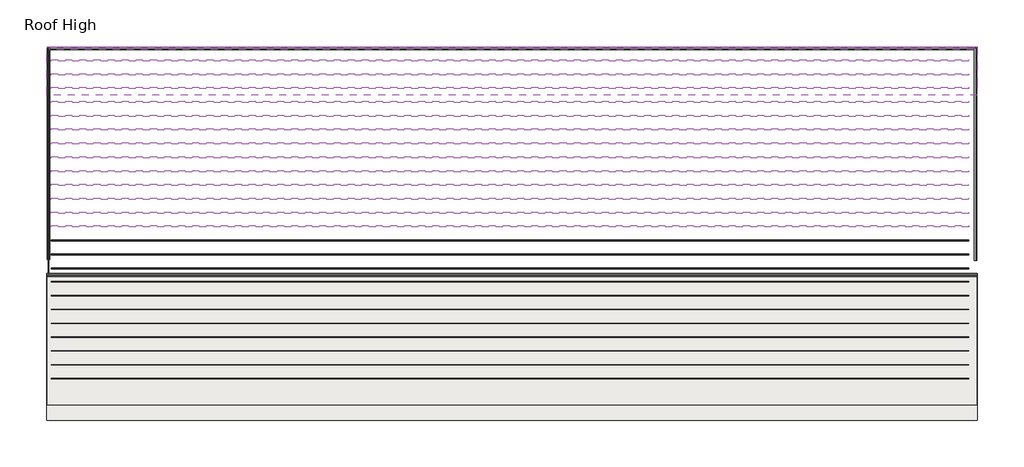
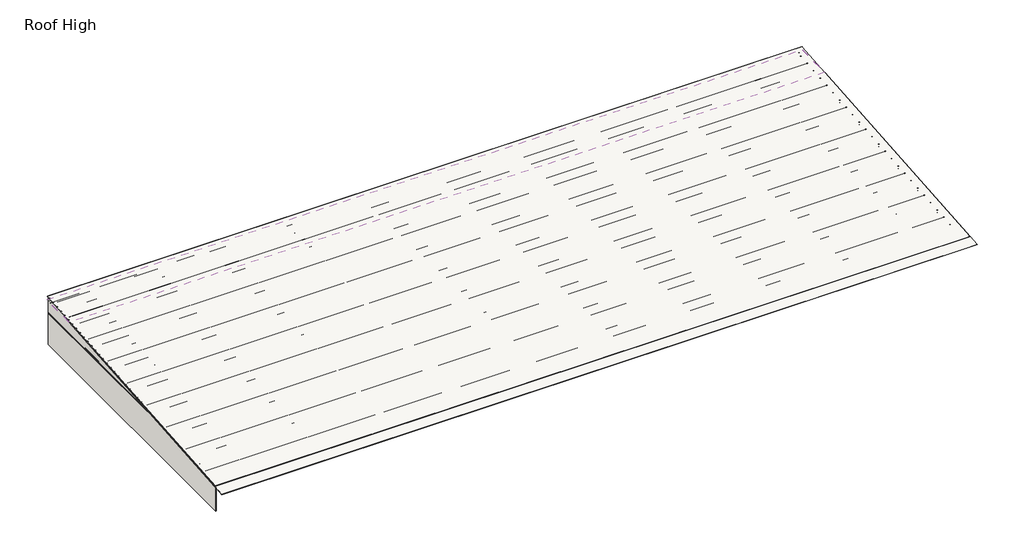
# One storey: 28 beams, 4 roofs, 1 proxy, 1 wall.
"""IFC4 building model written with IfcOpenShell, lengths in millimetres."""

import ifcopenshell
import ifcopenshell.guid

model = None  # the IFC model being written
_history = None  # IfcOwnerHistory: only IFC2X3 demands one
_inside = {}  # id of a spatial element -> (the spatial element, [elements in it])
_under = {}  # id of a project, library or spatial element -> (it, [spatial elements below it])
_declared = {}  # id of a project -> (the project, [libraries it declares])
_typed = {}  # id of a type object -> (the type object, [elements of that type])
_made_of = {}  # id of a material, layer set ... -> (it, [elements and type objects made of it])


def new_model(schema):
    """Start an empty IFC model of exactly this schema.

    Asked for "IFC4X3", IfcOpenShell would pick the latest addendum, in which some entities
    have other attributes; the version numbers below select the first issue.
    IFC2X3 requires an IfcOwnerHistory on every rooted entity: one is made here for all.
    """
    global model, _history
    if schema == "IFC4X3":
        model = ifcopenshell.file(schema_version=(4, 3, 0, 0))
    else:
        model = ifcopenshell.file(schema=schema)
    _inside.clear()
    _under.clear()
    _declared.clear()
    _typed.clear()
    _made_of.clear()
    _history = None
    if model.schema == "IFC2X3":
        org = make("IfcOrganization", Name="unknown")
        user = make(
            "IfcPersonAndOrganization",
            ThePerson=make("IfcPerson", FamilyName="unknown"),
            TheOrganization=org,
        )
        app = make(
            "IfcApplication",
            ApplicationDeveloper=org,
            Version="unknown",
            ApplicationFullName="unknown",
            ApplicationIdentifier="unknown",
        )
        _history = make(
            "IfcOwnerHistory",
            OwningUser=user,
            OwningApplication=app,
            ChangeAction="ADDED",
            CreationDate=0,
        )
    return model


def make(cls, **values):
    """One entity of the class cls with the attributes given. An attribute that is None is left unset."""
    return model.create_entity(
        cls, **{name: value for name, value in values.items() if value is not None}
    )


def rooted(cls, **values):
    """An entity with a GlobalId (a new one), such as an element, a storey or a relation."""
    return make(cls, GlobalId=ifcopenshell.guid.new(), OwnerHistory=_history, **values)


def si_unit(unit_type, name, prefix=None):
    """IfcSIUnit, for example si_unit("LENGTHUNIT", "METRE", prefix="MILLI")."""
    return make("IfcSIUnit", UnitType=unit_type, Prefix=prefix, Name=name)


def assignment(units):
    """IfcUnitAssignment: the units of a project."""
    return None if units is None else make("IfcUnitAssignment", Units=units)


def point(xyz):
    """IfcCartesianPoint."""
    return None if xyz is None else make("IfcCartesianPoint", Coordinates=xyz)


def direction(xyz):
    """IfcDirection."""
    return None if xyz is None else make("IfcDirection", DirectionRatios=xyz)


def frame(location, z_axis=None, x_axis=None):
    """IfcAxis2Placement3D, a coordinate frame: its origin and axes. An axis left out is left unset."""
    return make(
        "IfcAxis2Placement3D",
        Location=point(location),
        Axis=direction(z_axis),
        RefDirection=direction(x_axis),
    )


def frame_2d(location, x_axis=None):
    """IfcAxis2Placement2D, a coordinate frame in the plane: its origin and x axis."""
    return make(
        "IfcAxis2Placement2D", Location=point(location), RefDirection=direction(x_axis)
    )


def origin():
    """The frame at (0, 0, 0) with its axes left unset."""
    return frame((0.0, 0.0, 0.0))


def place(relative_to, where):
    """IfcLocalPlacement: puts the frame where relative to a parent placement (None: the world)."""
    return make(
        "IfcLocalPlacement", PlacementRelTo=relative_to, RelativePlacement=where
    )


def context(
    kind, dimensions, precision=None, world=None, true_north=None, identifier=None
):
    """IfcGeometricRepresentationContext, for example the 3D "Model" context."""
    return make(
        "IfcGeometricRepresentationContext",
        ContextIdentifier=identifier,
        ContextType=kind,
        CoordinateSpaceDimension=dimensions,
        Precision=precision,
        WorldCoordinateSystem=world,
        TrueNorth=true_north,
    )


def project(units=None, contexts=None):
    """IfcProject with its units and contexts."""
    return rooted(
        "IfcProject",
        Name="project",
        RepresentationContexts=contexts,
        UnitsInContext=assignment(units),
    )


def spatial(cls, under=None, at=None, **own):
    """A site, building, storey or space (cls), placed at a placement, below another one or the project."""
    s = rooted(cls, ObjectPlacement=at, **own)
    if under is not None:
        _under.setdefault(under.id(), (under, []))[1].append(s)
    return s


def polyline(points):
    """IfcPolyline through the points."""
    return make("IfcPolyline", Points=[point(p) for p in points])


def circle_curve(where, radius):
    """IfcCircle in the frame where."""
    return make("IfcCircle", Position=where, Radius=radius)


def trimmed(basis, trim1, trim2, sense, master):
    """IfcTrimmedCurve: the piece of a basis curve between two trims."""
    return make(
        "IfcTrimmedCurve",
        BasisCurve=basis,
        Trim1=trim1,
        Trim2=trim2,
        SenseAgreement=sense,
        MasterRepresentation=master,
    )


def segment(curve, same_sense, transition):
    """IfcCompositeCurveSegment."""
    return make(
        "IfcCompositeCurveSegment",
        Transition=transition,
        SameSense=same_sense,
        ParentCurve=curve,
    )


def composite_curve(segments, self_intersect=None):
    """IfcCompositeCurve: segments joined end to end."""
    return make("IfcCompositeCurve", Segments=segments, SelfIntersect=self_intersect)


def outline(outer, holes=None, kind="AREA"):
    """IfcArbitraryClosedProfileDef: a profile drawn as a closed curve; with holes, ...WithVoids."""
    if holes is None:
        return make("IfcArbitraryClosedProfileDef", ProfileType=kind, OuterCurve=outer)
    return make(
        "IfcArbitraryProfileDefWithVoids",
        ProfileType=kind,
        OuterCurve=outer,
        InnerCurves=holes,
    )


def extrude(swept, where, along, depth):
    """IfcExtrudedAreaSolid: the profile swept, set in the frame where, extruded along a direction by depth."""
    return make(
        "IfcExtrudedAreaSolid",
        SweptArea=swept,
        Position=where,
        ExtrudedDirection=direction(along),
        Depth=depth,
    )


def faces_of(points, faces, orient=None, outer=None):
    """IfcFace entities. A face is a list of loops; a loop is a list of indices into points, from 0.

    orient and outer hold one flag for each loop. By default every Orientation is true, the
    first loop of a face is its IfcFaceOuterBound and the others are IfcFaceBound.
    """
    made = []
    for i, loops in enumerate(faces):
        bounds = []
        for j, loop in enumerate(loops):
            is_outer = j == 0 if outer is None else outer[i][j]
            bounds.append(
                make(
                    "IfcFaceOuterBound" if is_outer else "IfcFaceBound",
                    Bound=make("IfcPolyLoop", Polygon=[points[k] for k in loop]),
                    Orientation=True if orient is None else orient[i][j],
                )
            )
        made.append(make("IfcFace", Bounds=bounds))
    return made


def faceted_brep(points, faces, orient=None, outer=None, voids=None):
    """IfcFacetedBrep: a solid bounded by flat faces; with voids (closed shells), ...WithVoids."""
    shared = [point(p) for p in points]
    hull = make("IfcClosedShell", CfsFaces=faces_of(shared, faces, orient, outer))
    if voids is None:
        return make("IfcFacetedBrep", Outer=hull)
    return make(
        "IfcFacetedBrepWithVoids",
        Outer=hull,
        Voids=[
            make(cls, CfsFaces=faces_of(shared, fs, o, b)) for cls, fs, o, b in voids
        ],
    )


def shape(context_of_items, identifier, shape_type, items):
    """IfcShapeRepresentation: the items that make up one representation, for example the "Body"."""
    return make(
        "IfcShapeRepresentation",
        ContextOfItems=context_of_items,
        RepresentationIdentifier=identifier,
        RepresentationType=shape_type,
        Items=items,
    )


def source(mapping_origin, context_of_items, identifier, shape_type, items):
    """IfcRepresentationMap: a shape defined once, which mapped items show again and again."""
    return make(
        "IfcRepresentationMap",
        MappingOrigin=mapping_origin,
        MappedRepresentation=shape(context_of_items, identifier, shape_type, items),
    )


def transform(
    local_origin,
    x_axis=None,
    y_axis=None,
    z_axis=None,
    scale=None,
    scale2=None,
    scale3=None,
    uniform=True,
):
    """IfcCartesianTransformationOperator3D, or its non-uniform kind. x_axis, y_axis, z_axis: its Axis1, 2, 3."""
    if uniform:
        return make(
            "IfcCartesianTransformationOperator3D",
            Axis1=direction(x_axis),
            Axis2=direction(y_axis),
            LocalOrigin=point(local_origin),
            Scale=scale,
            Axis3=direction(z_axis),
        )
    return make(
        "IfcCartesianTransformationOperator3DnonUniform",
        Axis1=direction(x_axis),
        Axis2=direction(y_axis),
        LocalOrigin=point(local_origin),
        Scale=scale,
        Axis3=direction(z_axis),
        Scale2=scale2,
        Scale3=scale3,
    )


def mapped(mapping_source, mapping_target):
    """IfcMappedItem: shows the shape of a source again, moved by a transform."""
    return make(
        "IfcMappedItem", MappingSource=mapping_source, MappingTarget=mapping_target
    )


def made_of(thing, what):
    """Note that an element or type object is made of a material, layer set ...; save() writes the relation."""
    if what is not None:
        _made_of.setdefault(what.id(), (what, []))[1].append(thing)
    return thing


def element(
    cls,
    number,
    at=None,
    inside=None,
    cuts=None,
    type_object=None,
    material=None,
    context=None,
    identifier="Body",
    shape_type=None,
    held_by="IfcProductDefinitionShape",
    body=None,
    shapes=None,
    **own,
):
    """One element of the class cls, such as IfcWall. Its Tag is "e" and its number.

    at: its placement. inside: the storey or other place that contains it. cuts: it is an
    opening in that element (IfcRelVoidsElement). A single representation is given by context,
    identifier, shape_type and body (its items); several are given by shapes. held_by: the class
    of the entity that holds the representations. save() writes the other relations.
    """
    e = rooted(cls, Tag="e%d" % number, ObjectPlacement=at, **own)
    if body is not None:
        shapes = [shape(context, identifier, shape_type, body)]
    if shapes is not None:
        e.Representation = make(held_by, Representations=shapes)
    if inside is not None:
        _inside.setdefault(inside.id(), (inside, []))[1].append(e)
    if cuts is not None:
        rooted(
            "IfcRelVoidsElement", RelatingBuildingElement=cuts, RelatedOpeningElement=e
        )
    if type_object is not None:
        _typed.setdefault(type_object.id(), (type_object, []))[1].append(e)
    return made_of(e, material)


def aggregate(whole, parts):
    """IfcRelAggregates: a whole, such as a stair, and the parts it consists of."""
    return rooted("IfcRelAggregates", RelatingObject=whole, RelatedObjects=parts)


def save(model, path):
    """Write the relations noted so far, then the file.

    IfcRelAggregates (storeys below a building ...), IfcRelContainedInSpatialStructure (elements
    in a storey), IfcRelDefinesByType, IfcRelAssociatesMaterial and IfcRelDeclares: one each for
    every whole, place, type object, material and project.
    """
    for whole, parts in _under.values():
        aggregate(whole, parts)
    for where, things in _inside.values():
        rooted(
            "IfcRelContainedInSpatialStructure",
            RelatedElements=things,
            RelatingStructure=where,
        )
    for kind, things in _typed.values():
        rooted("IfcRelDefinesByType", RelatedObjects=things, RelatingType=kind)
    for what, things in _made_of.values():
        rooted("IfcRelAssociatesMaterial", RelatedObjects=things, RelatingMaterial=what)
    for by, libraries in _declared.values():
        rooted("IfcRelDeclares", RelatingContext=by, RelatedDefinitions=libraries)
    model.write(path)


def beam_2a24e19f(model_context):
    return source(origin(), model_context, "Body", "SweptSolid", [
        extrude(outline(composite_curve([segment(polyline([(63.5, 127.0), (75.745104, 112.4068534), (73.6169367, 110.621109), (62.204539, 124.221875), (3.3005807, 124.221875)]), True, "CONTINUOUS"), segment(trimmed(circle_curve(frame_2d((3.3741066, 122.2381931)), 1.9850441), [point((3.3005807, 124.221875))], [point((1.3890625, 122.2381931))], True, "CARTESIAN"), True, "CONTINUOUS"), segment(polyline([(1.3890625, 122.2381931), (1.3890625, -122.2375)]), True, "CONTINUOUS"), segment(trimmed(circle_curve(frame_2d((-3.3734375, -122.2375)), 4.7625), [point((1.3890625, -122.2375))], [point((-3.3734375, -127.0))], False, "CARTESIAN"), True, "CONTINUOUS"), segment(polyline([(-3.3734375, -127.0), (-63.5, -127.0), (-75.745104, -112.4068534), (-73.6169367, -110.621109), (-62.204539, -124.221875), (-3.2694106, -124.221875)]), True, "CONTINUOUS"), segment(trimmed(circle_curve(frame_2d((-3.3748024, -122.2389339)), 1.9857399), [point((-3.2694106, -124.221875))], [point((-1.3890625, -122.2389339))], True, "CARTESIAN"), True, "CONTINUOUS"), segment(polyline([(-1.3890625, -122.2389339), (-1.3890625, 122.2375)]), True, "CONTINUOUS"), segment(trimmed(circle_curve(frame_2d((3.3734375, 122.2375)), 4.7625), [point((-1.3890625, 122.2375))], [point((3.3734375, 127.0))], False, "CARTESIAN"), True, "CONTINUOUS"), segment(polyline([(3.3734375, 127.0), (63.5, 127.0)]), True, "CONTINUOUS")], self_intersect=False)), frame((-40373.3, 0.0, 0.0), z_axis=(1.0, 0.0, 0.0), x_axis=(0.0, 1.0, 0.0)), (0.0, 0.0, 1.0), 80505.2999999),
    ])


def beam_abf8bc6d(model_context):
    return source(origin(), model_context, "Body", "SweptSolid", [
        extrude(outline(composite_curve([segment(polyline([(63.5, 127.0), (75.745104, 112.4068534), (73.6169367, 110.621109), (62.204539, 124.221875), (3.3005807, 124.221875)]), True, "CONTINUOUS"), segment(trimmed(circle_curve(frame_2d((3.3741066, 122.2381931)), 1.9850441), [point((3.3005807, 124.221875))], [point((1.3890625, 122.2381931))], True, "CARTESIAN"), True, "CONTINUOUS"), segment(polyline([(1.3890625, 122.2381931), (1.3890625, -122.2375)]), True, "CONTINUOUS"), segment(trimmed(circle_curve(frame_2d((-3.3734375, -122.2375)), 4.7625), [point((1.3890625, -122.2375))], [point((-3.3734375, -127.0))], False, "CARTESIAN"), True, "CONTINUOUS"), segment(polyline([(-3.3734375, -127.0), (-63.5, -127.0), (-75.745104, -112.4068534), (-73.6169367, -110.621109), (-62.204539, -124.221875), (-3.2694106, -124.221875)]), True, "CONTINUOUS"), segment(trimmed(circle_curve(frame_2d((-3.3748024, -122.2389339)), 1.9857399), [point((-3.2694106, -124.221875))], [point((-1.3890625, -122.2389339))], True, "CARTESIAN"), True, "CONTINUOUS"), segment(polyline([(-1.3890625, -122.2389339), (-1.3890625, 122.2375)]), True, "CONTINUOUS"), segment(trimmed(circle_curve(frame_2d((3.3734375, 122.2375)), 4.7625), [point((-1.3890625, 122.2375))], [point((3.3734375, 127.0))], False, "CARTESIAN"), True, "CONTINUOUS"), segment(polyline([(3.3734375, 127.0), (63.5, 127.0)]), True, "CONTINUOUS")], self_intersect=False)), frame((-40373.3, 0.0, 0.0), z_axis=(1.0, 0.0, 0.0), x_axis=(0.0, 1.0, 0.0)), (0.0, 0.0, 1.0), 80505.3),
    ])


def beam_1069c96b(model_context):
    return source(origin(), model_context, "Body", "SweptSolid", [
        extrude(outline(composite_curve([segment(polyline([(-63.5, 101.6), (-3.3734375, 101.6)]), True, "CONTINUOUS"), segment(trimmed(circle_curve(frame_2d((-3.3734375, 96.8375)), 4.7625), [point((-3.3734375, 101.6))], [point((1.3890625, 96.8375))], False, "CARTESIAN"), True, "CONTINUOUS"), segment(polyline([(1.3890625, 96.8375), (1.3890625, -96.8389339)]), True, "CONTINUOUS"), segment(trimmed(circle_curve(frame_2d((3.3748024, -96.8389339)), 1.9857399), [point((1.3890625, -96.8389339))], [point((3.2694106, -98.821875))], True, "CARTESIAN"), True, "CONTINUOUS"), segment(polyline([(3.2694106, -98.821875), (62.204539, -98.821875), (73.6169367, -85.221109), (75.745104, -87.0068534), (63.5, -101.6), (3.3734375, -101.6)]), True, "CONTINUOUS"), segment(trimmed(circle_curve(frame_2d((3.3734375, -96.8375)), 4.7625), [point((3.3734375, -101.6))], [point((-1.3890625, -96.8375))], False, "CARTESIAN"), True, "CONTINUOUS"), segment(polyline([(-1.3890625, -96.8375), (-1.3890625, 96.8381931)]), True, "CONTINUOUS"), segment(trimmed(circle_curve(frame_2d((-3.3741066, 96.8381931)), 1.9850441), [point((-1.3890625, 96.8381931))], [point((-3.3005807, 98.821875))], True, "CARTESIAN"), True, "CONTINUOUS"), segment(polyline([(-3.3005807, 98.821875), (-62.204539, 98.821875), (-73.6169367, 85.221109), (-75.745104, 87.0068534), (-63.5, 101.6)]), True, "CONTINUOUS")], self_intersect=False)), frame((-40602.569726, 0.0, 0.0), z_axis=(1.0, 0.0, 0.0), x_axis=(0.0, 1.0, 0.0)), (0.0, 0.0, 1.0), 81057.5019525),
    ])


def beam_935b8cdd(model_context):
    return source(origin(), model_context, "Body", "SweptSolid", [
        extrude(outline(composite_curve([segment(polyline([(63.5, 101.6), (75.745104, 87.0068534), (73.6169367, 85.221109), (62.204539, 98.821875), (3.3005807, 98.821875)]), True, "CONTINUOUS"), segment(trimmed(circle_curve(frame_2d((3.3741066, 96.8381931)), 1.9850441), [point((3.3005807, 98.821875))], [point((1.3890625, 96.8381931))], True, "CARTESIAN"), True, "CONTINUOUS"), segment(polyline([(1.3890625, 96.8381931), (1.3890625, -96.8375)]), True, "CONTINUOUS"), segment(trimmed(circle_curve(frame_2d((-3.3734375, -96.8375)), 4.7625), [point((1.3890625, -96.8375))], [point((-3.3734375, -101.6))], False, "CARTESIAN"), True, "CONTINUOUS"), segment(polyline([(-3.3734375, -101.6), (-63.5, -101.6), (-75.745104, -87.0068534), (-73.6169367, -85.221109), (-62.204539, -98.821875), (-3.2694106, -98.821875)]), True, "CONTINUOUS"), segment(trimmed(circle_curve(frame_2d((-3.3748024, -96.8389339)), 1.9857399), [point((-3.2694106, -98.821875))], [point((-1.3890625, -96.8389339))], True, "CARTESIAN"), True, "CONTINUOUS"), segment(polyline([(-1.3890625, -96.8389339), (-1.3890625, 96.8375)]), True, "CONTINUOUS"), segment(trimmed(circle_curve(frame_2d((3.3734375, 96.8375)), 4.7625), [point((-1.3890625, 96.8375))], [point((3.3734375, 101.6))], False, "CARTESIAN"), True, "CONTINUOUS"), segment(polyline([(3.3734375, 101.6), (63.5, 101.6)]), True, "CONTINUOUS")], self_intersect=False)), frame((-9323.6355469, 0.0, 0.0), z_axis=(1.0, 0.0, 0.0), x_axis=(0.0, 1.0, 0.0)), (0.0, 0.0, 1.0), 18647.2710937),
    ])


def beam_7c8f2e1c(model_context):
    return source(origin(), model_context, "Body", "SweptSolid", [
        extrude(outline(composite_curve([segment(polyline([(-63.5, 101.6), (-3.3734375, 101.6)]), True, "CONTINUOUS"), segment(trimmed(circle_curve(frame_2d((-3.3734375, 96.8375)), 4.7625), [point((-3.3734375, 101.6))], [point((1.3890625, 96.8375))], False, "CARTESIAN"), True, "CONTINUOUS"), segment(polyline([(1.3890625, 96.8375), (1.3890625, -96.8389339)]), True, "CONTINUOUS"), segment(trimmed(circle_curve(frame_2d((3.3748024, -96.8389339)), 1.9857399), [point((1.3890625, -96.8389339))], [point((3.2694106, -98.821875))], True, "CARTESIAN"), True, "CONTINUOUS"), segment(polyline([(3.2694106, -98.821875), (62.204539, -98.821875), (73.6169367, -85.221109), (75.745104, -87.0068534), (63.5, -101.6), (3.3734375, -101.6)]), True, "CONTINUOUS"), segment(trimmed(circle_curve(frame_2d((3.3734375, -96.8375)), 4.7625), [point((3.3734375, -101.6))], [point((-1.3890625, -96.8375))], False, "CARTESIAN"), True, "CONTINUOUS"), segment(polyline([(-1.3890625, -96.8375), (-1.3890625, 96.8381931)]), True, "CONTINUOUS"), segment(trimmed(circle_curve(frame_2d((-3.3741066, 96.8381931)), 1.9850441), [point((-1.3890625, 96.8381931))], [point((-3.3005807, 98.821875))], True, "CARTESIAN"), True, "CONTINUOUS"), segment(polyline([(-3.3005807, 98.821875), (-62.204539, 98.821875), (-73.6169367, 85.221109), (-75.745104, 87.0068534), (-63.5, 101.6)]), True, "CONTINUOUS")], self_intersect=False)), frame((-9209.8316406, 0.0, 0.0), z_axis=(1.0, 0.0, 0.0), x_axis=(0.0, 1.0, 0.0)), (0.0, 0.0, 1.0), 18529.7960937),
    ])


def beam_4e68f0c2(model_context):
    return source(origin(), model_context, "Body", "SweptSolid", [
        extrude(outline(composite_curve([segment(polyline([(-63.5, 101.6), (-3.3734375, 101.6)]), True, "CONTINUOUS"), segment(trimmed(circle_curve(frame_2d((-3.3734375, 96.8375)), 4.7625), [point((-3.3734375, 101.6))], [point((1.3890625, 96.8375))], False, "CARTESIAN"), True, "CONTINUOUS"), segment(polyline([(1.3890625, 96.8375), (1.3890625, -96.8389339)]), True, "CONTINUOUS"), segment(trimmed(circle_curve(frame_2d((3.3748024, -96.8389339)), 1.9857399), [point((1.3890625, -96.8389339))], [point((3.2694106, -98.821875))], True, "CARTESIAN"), True, "CONTINUOUS"), segment(polyline([(3.2694106, -98.821875), (62.204539, -98.821875), (73.6169367, -85.221109), (75.745104, -87.0068534), (63.5, -101.6), (3.3734375, -101.6)]), True, "CONTINUOUS"), segment(trimmed(circle_curve(frame_2d((3.3734375, -96.8375)), 4.7625), [point((3.3734375, -101.6))], [point((-1.3890625, -96.8375))], False, "CARTESIAN"), True, "CONTINUOUS"), segment(polyline([(-1.3890625, -96.8375), (-1.3890625, 96.8381931)]), True, "CONTINUOUS"), segment(trimmed(circle_curve(frame_2d((-3.3741066, 96.8381931)), 1.9850441), [point((-1.3890625, 96.8381931))], [point((-3.3005807, 98.821875))], True, "CARTESIAN"), True, "CONTINUOUS"), segment(polyline([(-3.3005807, 98.821875), (-62.204539, 98.821875), (-73.6169367, 85.221109), (-75.745104, 87.0068534), (-63.5, 101.6)]), True, "CONTINUOUS")], self_intersect=False)), frame((-40615.2697266, 0.0, 0.0), z_axis=(1.0, 0.0, 0.0), x_axis=(0.0, 1.0, 0.0)), (0.0, 0.0, 1.0), 81070.2019531),
    ])


model = new_model("IFC4")

# Units and contexts
model_context = context("Model", 3, world=origin())
ifc_project = project(units=[si_unit("LENGTHUNIT", "METRE", prefix="MILLI")], contexts=[model_context])

# Site, building, storey
site = spatial("IfcSite", under=ifc_project)
building = spatial("IfcBuilding", under=site)
storey = spatial("IfcBuildingStorey", under=building, Name="Roof High", Elevation=8737.6)

# Beams
placement = place(None, origin())
beam_shape = beam_2a24e19f(model_context)
element("IfcBeam", 1, ObjectType="Girt_Z : 10\"D", at=placement, inside=storey, context=model_context, shape_type="MappedRepresentation", body=[
    mapped(beam_shape, transform((619401.6117241, -537915.7766687, 11367.5039356), x_axis=(1.0, 0.0, 0.0), y_axis=(0.0, 0.996545758244879, 0.08304547985374816), z_axis=(0.0, -0.08304547985374816, 0.996545758244879))),
])
element("IfcBeam", 2, ObjectType="Girt_Z : 10\"D", at=placement, inside=storey, context=model_context, shape_type="MappedRepresentation", body=[
    mapped(beam_shape, transform((619401.6117241, -539130.7652571, 11266.2548865), x_axis=(1.0, 0.0, 0.0), y_axis=(0.0, 0.996545758244879, 0.08304547985374816), z_axis=(0.0, -0.08304547985374816, 0.996545758244879))),
])
element("IfcBeam", 3, ObjectType="Girt_Z : 10\"D", at=placement, inside=storey, context=model_context, shape_type="MappedRepresentation", body=[
    mapped(beam_shape, transform((619401.6117241, -540345.7538456, 11165.0058375), x_axis=(1.0, 0.0, 0.0), y_axis=(0.0, 0.996545758244879, 0.08304547985374816), z_axis=(0.0, -0.08304547985374816, 0.996545758244879))),
])
element("IfcBeam", 4, ObjectType="Girt_Z : 10\"D", at=placement, inside=storey, context=model_context, shape_type="MappedRepresentation", body=[
    mapped(beam_shape, transform((619401.6117241, -541560.742434, 11063.7567885), x_axis=(1.0, 0.0, 0.0), y_axis=(0.0, 0.996545758244879, 0.08304547985374816), z_axis=(0.0, -0.08304547985374816, 0.996545758244879))),
])
element("IfcBeam", 5, ObjectType="Girt_Z : 10\"D", at=placement, inside=storey, context=model_context, shape_type="MappedRepresentation", body=[
    mapped(beam_shape, transform((619401.6117241, -542775.7310225, 10962.5077394), x_axis=(1.0, 0.0, 0.0), y_axis=(0.0, 0.996545758244879, 0.08304547985374816), z_axis=(0.0, -0.08304547985374816, 0.996545758244879))),
])
element("IfcBeam", 6, ObjectType="Girt_Z : 10\"D", at=placement, inside=storey, context=model_context, shape_type="MappedRepresentation", body=[
    mapped(beam_shape, transform((619401.6117241, -543990.7196109, 10861.2586904), x_axis=(1.0, 0.0, 0.0), y_axis=(0.0, 0.996545758244879, 0.08304547985374816), z_axis=(0.0, -0.08304547985374816, 0.996545758244879))),
])
element("IfcBeam", 7, ObjectType="Girt_Z : 10\"D", at=placement, inside=storey, context=model_context, shape_type="MappedRepresentation", body=[
    mapped(beam_shape, transform((619401.6117241, -545205.7081994, 10760.0096414), x_axis=(1.0, 0.0, 0.0), y_axis=(0.0, 0.996545758244879, 0.08304547985374816), z_axis=(0.0, -0.08304547985374816, 0.996545758244879))),
])
element("IfcBeam", 8, ObjectType="Girt_Z : 10\"D", at=placement, inside=storey, context=model_context, shape_type="MappedRepresentation", body=[
    mapped(beam_shape, transform((619401.6117241, -546420.6967878, 10658.7605923), x_axis=(1.0, 0.0, 0.0), y_axis=(0.0, 0.996545758244879, 0.08304547985374816), z_axis=(0.0, -0.08304547985374816, 0.996545758244879))),
])
element("IfcBeam", 9, ObjectType="Girt_Z : 10\"D", at=placement, inside=storey, context=model_context, shape_type="MappedRepresentation", body=[
    mapped(beam_shape, transform((619401.6117241, -547635.6853763, 10557.5115433), x_axis=(1.0, 0.0, 0.0), y_axis=(0.0, 0.996545758244879, 0.08304547985374816), z_axis=(0.0, -0.08304547985374816, 0.996545758244879))),
])
element("IfcBeam", 10, ObjectType="Girt_Z : 10\"D", at=placement, inside=storey, context=model_context, shape_type="MappedRepresentation", body=[
    mapped(beam_shape, transform((619401.6117241, -548850.6739647, 10456.2624942), x_axis=(1.0, 0.0, 0.0), y_axis=(0.0, 0.996545758244879, 0.08304547985374816), z_axis=(0.0, -0.08304547985374816, 0.996545758244879))),
])
element("IfcBeam", 11, ObjectType="Girt_Z : 10\"D", at=placement, inside=storey, context=model_context, shape_type="MappedRepresentation", body=[
    mapped(beam_shape, transform((619401.6117241, -550065.6625532, 10355.0134452), x_axis=(1.0, 0.0, 0.0), y_axis=(0.0, 0.996545758244879, 0.08304547985374816), z_axis=(0.0, -0.08304547985374816, 0.996545758244879))),
])
element("IfcBeam", 12, ObjectType="Girt_Z : 10\"D", at=placement, inside=storey, context=model_context, shape_type="MappedRepresentation", body=[
    mapped(beam_shape, transform((619401.6117241, -551280.6511416, 10253.7643962), x_axis=(1.0, 0.0, 0.0), y_axis=(0.0, 0.996545758244879, 0.08304547985374816), z_axis=(0.0, -0.08304547985374816, 0.996545758244879))),
])
element("IfcBeam", 13, ObjectType="Girt_Z : 10\"D", at=placement, inside=storey, context=model_context, shape_type="MappedRepresentation", body=[
    mapped(beam_shape, transform((619401.6117241, -552495.6397301, 10152.5153471), x_axis=(1.0, 0.0, 0.0), y_axis=(0.0, 0.996545758244879, 0.08304547985374816), z_axis=(0.0, -0.08304547985374816, 0.996545758244879))),
])
element("IfcBeam", 14, ObjectType="Girt_Z : 10\"D", at=placement, inside=storey, context=model_context, shape_type="MappedRepresentation", body=[
    mapped(beam_shape, transform((619401.6117241, -553710.6283185, 10051.2662981), x_axis=(1.0, 0.0, 0.0), y_axis=(0.0, 0.996545758244879, 0.08304547985374816), z_axis=(0.0, -0.08304547985374816, 0.996545758244879))),
])
element("IfcBeam", 15, ObjectType="Girt_Z : 10\"D", at=placement, inside=storey, context=model_context, shape_type="MappedRepresentation", body=[
    mapped(beam_shape, transform((619401.6117241, -554925.616907, 9950.0172491), x_axis=(1.0, 0.0, 0.0), y_axis=(0.0, 0.996545758244879, 0.08304547985374816), z_axis=(0.0, -0.08304547985374816, 0.996545758244879))),
])
element("IfcBeam", 16, ObjectType="Girt_Z : 10\"D", at=placement, inside=storey, context=model_context, shape_type="MappedRepresentation", body=[
    mapped(beam_shape, transform((619401.6117241, -556140.6054954, 9848.7682), x_axis=(1.0, 0.0, 0.0), y_axis=(0.0, 0.996545758244879, 0.08304547985374816), z_axis=(0.0, -0.08304547985374816, 0.996545758244879))),
])
element("IfcBeam", 17, ObjectType="Girt_Z : 10\"D", at=placement, inside=storey, context=model_context, shape_type="MappedRepresentation", body=[
    mapped(beam_shape, transform((619401.6117241, -557355.5940839, 9747.519151), x_axis=(1.0, 0.0, 0.0), y_axis=(0.0, 0.996545758244879, 0.08304547985374816), z_axis=(0.0, -0.08304547985374816, 0.996545758244879))),
])
element("IfcBeam", 18, ObjectType="Girt_Z : 10\"D", at=placement, inside=storey, context=model_context, shape_type="MappedRepresentation", body=[
    mapped(beam_shape, transform((619401.6117241, -558570.5826724, 9646.2701019), x_axis=(1.0, 0.0, 0.0), y_axis=(0.0, 0.996545758244879, 0.08304547985374816), z_axis=(0.0, -0.08304547985374816, 0.996545758244879))),
])
element("IfcBeam", 19, ObjectType="Girt_Z : 10\"D", at=placement, inside=storey, context=model_context, shape_type="MappedRepresentation", body=[
    mapped(beam_shape, transform((619401.6117241, -559785.5712608, 9545.0210529), x_axis=(1.0, 0.0, 0.0), y_axis=(0.0, 0.996545758244879, 0.08304547985374816), z_axis=(0.0, -0.08304547985374816, 0.996545758244879))),
])
element("IfcBeam", 20, ObjectType="Girt_Z : 10\"D", at=placement, inside=storey, context=model_context, shape_type="MappedRepresentation", body=[
    mapped(beam_shape, transform((619401.6117241, -561000.5598493, 9443.7720039), x_axis=(1.0, 0.0, 0.0), y_axis=(0.0, 0.996545758244879, 0.08304547985374816), z_axis=(0.0, -0.08304547985374816, 0.996545758244879))),
])
beam_2_shape = beam_abf8bc6d(model_context)
element("IfcBeam", 21, ObjectType="Girt_Z : 10\"D", at=placement, inside=storey, context=model_context, shape_type="MappedRepresentation", body=[
    mapped(beam_2_shape, transform((619401.6117241, -562215.5484377, 9342.5229548), x_axis=(1.0, 0.0, 0.0), y_axis=(0.0, 0.996545758244879, 0.08304547985374816), z_axis=(0.0, -0.08304547985374816, 0.996545758244879))),
])
element("IfcBeam", 22, ObjectType="Girt_Z : 10\"D", at=placement, inside=storey, context=model_context, shape_type="MappedRepresentation", body=[
    mapped(beam_2_shape, transform((619401.6117241, -563430.5370262, 9241.2739058), x_axis=(1.0, 0.0, 0.0), y_axis=(0.0, 0.996545758244879, 0.08304547985374816), z_axis=(0.0, -0.08304547985374816, 0.996545758244879))),
])
element("IfcBeam", 23, ObjectType="Girt_Z : 10\"D", at=placement, inside=storey, context=model_context, shape_type="MappedRepresentation", body=[
    mapped(beam_2_shape, transform((619401.6117241, -564645.5256146, 9140.0248567), x_axis=(1.0, 0.0, 0.0), y_axis=(0.0, 0.996545758244879, 0.08304547985374816), z_axis=(0.0, -0.08304547985374816, 0.996545758244879))),
])
element("IfcBeam", 24, ObjectType="Girt_Z : 10\"D", at=placement, inside=storey, context=model_context, shape_type="MappedRepresentation", body=[
    mapped(beam_2_shape, transform((619401.6117241, -565860.5142031, 9038.7758077), x_axis=(1.0, 0.0, 0.0), y_axis=(0.0, 0.996545758244879, 0.08304547985374816), z_axis=(0.0, -0.08304547985374816, 0.996545758244879))),
])
beam_3_shape = beam_1069c96b(model_context)
element("IfcBeam", 25, ObjectType="Girt_Z : 8\"D", at=placement, inside=storey, context=model_context, shape_type="MappedRepresentation", body=[
    mapped(beam_3_shape, transform((619520.0044974, -536855.7413841, 9753.6), x_axis=(1.0000000000000002, 0.0, 0.0), y_axis=(0.0, 0.0, 1.0000000000000002), z_axis=(0.0, -1.0000000000000002, 0.0))),
])
beam_4_shape = beam_935b8cdd(model_context)
element("IfcBeam", 26, ObjectType="Girt_Z : 8\"D", at=placement, inside=storey, context=model_context, shape_type="MappedRepresentation", body=[
    mapped(beam_4_shape, transform((660105.1117239, -546179.376931, 9753.6), x_axis=(0.0, 1.0000000000000002, 0.0), y_axis=(0.0, 0.0, -1.0000000000000002), z_axis=(-1.0000000000000002, 0.0, 0.0))),
])
beam_5_shape = beam_7c8f2e1c(model_context)
element("IfcBeam", 27, ObjectType="Girt_Z : 8\"D", at=placement, inside=storey, context=model_context, shape_type="MappedRepresentation", body=[
    mapped(beam_5_shape, transform((578803.1347708, -546175.7058372, 9753.6), x_axis=(0.0, 1.0000000000000002, 0.0), y_axis=(0.0, 0.0, 1.0000000000000002), z_axis=(1.0000000000000002, 0.0, 0.0))),
])
beam_6_shape = beam_4e68f0c2(model_context)
element("IfcBeam", 28, ObjectType="Girt_Z : 8\"D", at=placement, inside=storey, context=model_context, shape_type="MappedRepresentation", body=[
    mapped(beam_6_shape, transform((619520.0044974, -536855.7413841, 10972.8), x_axis=(1.0000000000000002, 0.0, 0.0), y_axis=(0.0, 0.0, 1.0000000000000002), z_axis=(0.0, -1.0000000000000002, 0.0))),
])

# Proxy
element("IfcBuildingElementProxy", 29, Name="Wall Sweeps", at=placement, inside=storey, context=model_context, shape_type="SweptSolid", body=[
    extrude(outline(polyline([(-536747.7913841, 11605.3516632), (-536693.7909841, 11605.3516632), (-536693.7909841, 11533.3680632), (-536696.9659841, 11533.3680632), (-536696.9659841, 11534.9555632), (-536695.3784841, 11534.9555632), (-536695.3784841, 11603.7641632), (-536746.2038841, 11603.7641632), (-536746.2038841, 11514.9403632), (-536740.3872841, 11514.9403632), (-536740.3872841, 11519.7028632), (-536738.7997841, 11519.7028632), (-536738.7997841, 11513.3528632), (-536747.7913841, 11513.3528632), (-536747.7913841, 11605.3516632)])), frame((578766.7848054, 0.0, 0.0), z_axis=(1.0, 0.0, 0.0), x_axis=(0.0, 1.0, 0.0)), (0.0, 0.0, 1.0), 81475.5021585),
])

# Roofs
element("IfcRoof", 30, ObjectType="arcoPlus_6124_with_IR", at=placement, inside=storey, context=model_context, shape_type="SweptSolid", body=[
    extrude(outline(polyline([(-568168.5413949, 9002.8608333), (-536724.1414187, 11623.227498), (-536724.1414187, 11611.1804157), (-568168.5413949, 8990.813751), (-568168.5413949, 9002.8608333)])), frame((578668.83476, 0.0, 0.0), z_axis=(1.0, 0.0, 0.0), x_axis=(0.0, 1.0, 0.0)), (0.0, 0.0, 1.0), 81557.8769747),
])
element("IfcRoof", 31, ObjectType="arcoPlus_6124_with_IR", at=placement, inside=storey, context=model_context, shape_type="SweptSolid", body=[
    extrude(outline(polyline([(-568204.1165841, 8982.9629009), (-540960.9909841, 11253.2233675), (-540960.9909841, 11241.1762853), (-568204.1165841, 8970.9158186), (-568204.1165841, 8982.9629009)])), frame((578625.3347708, 0.0, 0.0), z_axis=(1.0, 0.0, 0.0), x_axis=(0.0, 1.0, 0.0)), (0.0, 0.0, 1.0), 81657.5769531),
])
element("IfcRoof", 32, ObjectType="Metal Roof - Structural Standing Seam", at=placement, inside=storey, context=model_context, shape_type="SweptSolid", body=[
    extrude(outline(polyline([(-540960.9909841, 11253.2233675), (-536693.7909841, 11608.8233675), (-536693.7909841, 11596.7762853), (-540960.9909841, 11241.1762853), (-540960.9909841, 11253.2233675)])), frame((578625.3347708, 0.0, 0.0), z_axis=(1.0, 0.0, 0.0), x_axis=(0.0, 1.0, 0.0)), (0.0, 0.0, 1.0), 81657.5769531),
])
element("IfcRoof", 33, ObjectType="Shading Material", at=placement, inside=storey, context=model_context, shape_type="SweptSolid", body=[
    extrude(outline(polyline([(-569520.1413841, 8873.2941675), (-568178.5413495, 8985.0941704), (-568178.5413495, 8973.0470881), (-569520.1413841, 8861.2470853), (-569520.1413841, 8873.2941675)])), frame((578625.3347708, 0.0, 0.0), z_axis=(1.0, 0.0, 0.0), x_axis=(0.0, 1.0, 0.0)), (0.0, 0.0, 1.0), 81657.5769531),
])

# Wall
element("IfcWall", 34, ObjectType="arcoPlus - 547", at=placement, inside=storey, context=model_context, shape_type="Brep", body=[
    faceted_brep([(578766.7848054, -536738.5661041, 6097.5875), (578766.7848054, -568164.1166641, 6097.5875), (578766.7848054, -568164.1166641, 8974.2491453), (578766.7848054, -536747.7913841, 11592.2762519), (578766.7848054, -536747.7913841, 11513.3528632), (578766.7848054, -536738.7997841, 11513.3528632), (578766.7848054, -536738.7997841, 11519.7028632), (578766.7848054, -536740.3872841, 11519.7028632), (578766.7848054, -536740.3872841, 11514.9403632), (578766.7848054, -536746.2038841, 11514.9403632), (578766.7848054, -536746.2038841, 11592.4085436), (578766.7848054, -536738.5661041, 11593.0450253), (578766.7848054, -536738.5661041, 11576.8528632), (578806.7847254, -568164.1166641, 6097.5875), (578806.7847254, -536738.5661041, 6097.5875), (578806.7847254, -536738.5661041, 11593.0450253), (578806.7847254, -536746.2038841, 11592.4085436), (578806.7847254, -536746.2038841, 11514.9403632), (578806.7847254, -536740.3872841, 11514.9403632), (578806.7847254, -536740.3872841, 11519.7028632), (578806.7847254, -536738.7997841, 11519.7028632), (578806.7847254, -536738.7997841, 11513.3528632), (578806.7847254, -536747.7913841, 11513.3528632), (578806.7847254, -536747.7913841, 11592.2762519), (578806.7847254, -568164.1166641, 8974.2491453)], [[[0, 1, 2, 3, 4, 5, 6, 7, 8, 9, 10, 11, 12]], [[13, 14, 15, 16, 17, 18, 19, 20, 21, 22, 23, 24]], [[2, 24, 23, 3]], [[15, 11, 10, 16]], [[1, 0, 14, 13]], [[24, 2, 1, 13]], [[11, 15, 14, 0, 12]], [[22, 4, 3, 23]], [[4, 22, 21, 5]], [[5, 21, 20, 6]], [[6, 20, 19, 7]], [[7, 19, 18, 8]], [[8, 18, 17, 9]], [[9, 17, 16, 10]]]),
])

save(model, "model.ifc")

# Revit data of these elements
# Project information
#   Project Issue Date = "Issue Date"
#   Project Status = "Project Status"
#   Client Name = "Xcel Fitness"
#   Project Address = "Enter address here"
#   Project Name = "Xcel Sports Complex"
#   Project Number = "Project Number"
# Grids (mm)
#   "1": line (579028.312, -472874.843) -> (579028.312, -580344.522)
#   "2": line (586368.912, -472874.843) -> (586368.912, -580344.522)
#   "3": line (593709.512, -472874.843) -> (593709.512, -580344.522)
#   "4": line (601050.112, -472874.843) -> (601050.112, -580344.522)
#   "5": line (608390.712, -472874.843) -> (608390.712, -580344.522)
#   "6": line (615731.312, -472874.843) -> (615731.312, -580344.522)
#   "7": line (623071.912, -472874.843) -> (623071.912, -580344.522)
#   "8": line (630412.512, -472874.843) -> (630412.512, -580344.522)
#   "9": line (637753.112, -472874.843) -> (637753.112, -580344.522)
#   "10": line (645093.712, -472874.843) -> (645093.712, -580344.522)
#   "11": line (652434.312, -472874.843) -> (652434.312, -580344.522)
#   "12": line (659774.912, -472874.843) -> (659774.912, -580344.522)
#   "I": line (499667.271, -578054.541) -> (746385.635, -578054.541)
#   "A": line (499667.271, -525019.341) -> (669398.695, -525019.341)
#   "D": line (499667.271, -543307.341) -> (669398.695, -543307.341)
#   "E": line (499667.271, -549403.341) -> (669398.695, -549403.341)
#   "F": line (499667.271, -555499.341) -> (669398.695, -555499.341)
#   "G": line (499667.271, -561595.341) -> (669398.695, -561595.341)
#   "B": line (499667.271, -531115.341) -> (669398.695, -531115.341)
#   "0": line (564347.112, -472874.843) -> (564347.112, -580344.522)
#   "0.2": line (568665.112, -472874.843) -> (568665.112, -580344.522)
#   "C": line (499667.271, -537211.341) -> (746385.635, -537211.341)
#   "H": line (499667.271, -567691.341) -> (746385.635, -567691.341)
#   "13": line (667115.512, -472874.843) -> (667115.512, -580344.522)
#   "H.5": line (499667.271, -575006.541) -> (746385.635, -575006.541)
# Type "Girt_Z : 10\"D"
#   Web_Thickness = 0' - 0 7/64"
#   Length [instance default] = 10' - 0"
#   Leg_1 = 0' - 2 1/2"
#   Height = 0' - 10"
#   Structural Material [instance default] = none
# Type "Girt_Z : 8\"D"
#   Web_Thickness = 0' - 0 7/64"
#   Length [instance default] = 10' - 0"
#   Leg_1 = 0' - 2 1/2"
#   Height = 0' - 8"
#   Structural Material [instance default] = none
# Type "arcoPlus_6124_with_IR"
#   Assembly Code = "B1020"
#   built-in parameter 1001600 = 0.039388 (stored number, unit not read)
#   Elevation_Transparency_Hack = 70
#   Layers, outside or top first: 0' - 0 121/256" "arcoPlus_6124_with_IR" (function 1)
# Type "Metal Roof - Structural Standing Seam"
#   Assembly Code = "B1020"
#   built-in parameter 1001600 = 0.039388 (stored number, unit not read)
#   Elevation_Transparency_Hack = 0
#   Layers, outside or top first: 0' - 0 121/256" "Metal Roof - Structural Standing Seam" (function 1)
# Type "Shading Material"
#   Assembly Code = "B1020"
#   built-in parameter 1001600 = 0.039388 (stored number, unit not read)
#   Elevation_Transparency_Hack = 0
#   Layers, outside or top first: 0' - 0 121/256" "Shading Material" (function 1)
# Type "arcoPlus - 547"
#   Assembly Code = "B2010"
#   Width = 0' - 1.5748"
#   Elevation_Transparency_Hack = 70
#   Layers, outside or top first: 0' - 1 147/256" "arcoPlus_324" (function 1)
# Elements 1, 2, 3, 4, 5, 6, 7, 8, 9, 10, 11, 12, 13, 14, 15, 16, 17, 18, 19, 20 (IfcBeam, "Girt_Z : 10\"D")
#   Structural Material = Steel
#   Structural Material = Steel
#   Phase Created = Phase 1
#   Materials on its faces: "Steel"
# Elements 21, 22, 23, 24 (IfcBeam, "Girt_Z : 10\"D")
#   Structural Material = none
#   Phase Created = Phase 1
# Elements 25, 26, 27, 28 (IfcBeam, "Girt_Z : 8\"D")
#   Comments = ""
#   Structural Material = Steel
#   Structural Material = Steel
#   Phase Created = Phase 1
#   Materials on its faces: "Steel"
# Element 29 (IfcBuildingElementProxy)
#   Phase Created = Phase 1
#   Materials on its faces: "Aluminum"
# Element 30 (IfcRoof, "arcoPlus_6124_with_IR")
#   OD_Option_2 = "N"
#   OD_Option_3 = "N"
#   OD_Option_4 = "N"
#   built-in parameter 1001705 = 38.1339 (stored number, unit not read)
#   built-in parameter 1001701 = 0.830754 (stored number, unit not read)
#   built-in parameter 1001710 = 33615
#   Phase Created = Phase 1
#   Materials on its faces: "arcoPlus_6124_with_IR"
# Element 31 (IfcRoof, "arcoPlus_6124_with_IR")
#   OD_Option_1 = "N"
#   OD_Option_2 = ""
#   OD_Option_3 = "N"
#   OD_Option_4 = "N"
#   built-in parameter 1001705 = 36.92 (stored number, unit not read)
#   built-in parameter 1001701 = 0.765472 (stored number, unit not read)
#   built-in parameter 1001710 = 33615
#   Phase Created = Phase 1
#   Materials on its faces: "arcoPlus_6124_with_IR"
# Element 32 (IfcRoof, "Metal Roof - Structural Standing Seam")
#   OD_Option_1 = "N"
#   OD_Option_2 = ""
#   OD_Option_3 = "N"
#   OD_Option_4 = "N"
#   built-in parameter 1001705 = 38.0867 (stored number, unit not read)
#   built-in parameter 1001701 = 8.21383 (stored number, unit not read)
#   built-in parameter 1001710 = 33615
#   Phase Created = Phase 1
#   Materials on its faces: "Metal Roof - Structural Standing Seam"
# Element 33 (IfcRoof, "Shading Material")
#   OD_Option_1 = "N"
#   OD_Option_2 = ""
#   OD_Option_3 = "N"
#   OD_Option_4 = "N"
#   built-in parameter 1001705 = 29.4787 (stored number, unit not read)
#   built-in parameter 1001701 = 0.405666 (stored number, unit not read)
#   built-in parameter 1001710 = 33615
#   Phase Created = Phase 1
#   Materials on its faces: "Shading Material"
# Element 34 (IfcWall, "arcoPlus - 547")
#   OD_Option_2 = "N"
#   OD_Option_3 = "N"
#   OD_Option_4 = "N"
#   built-in parameter 1001111 = -8' - 8"
#   Top Offset = 0' - 0"
#   Base Offset = -8' - 8"
#   Unconnected Height = 20' - 8"
#   wall height = 20' - 8"
#   Phase Created = Phase 1
#   Base Constraint = Roof High
#   Materials on its faces: "arcoPlus_324"
# Materials
#   "arcoPlus_6124_with_IR": class "Miscellaneous", colour RGB 196 196 196, transparency 0.3, Cost = 0
#   "Metal Roof - Structural Standing Seam": class "Generic", colour RGB 120 120 120, transparency 0, Cost = 0
#   "Shading Material": class "Generic", colour RGB 170 170 170, transparency 0, Cost = 0
#   "arcoPlus_324": class "Miscellaneous", colour RGB 197 197 197, transparency 0.3, Cost = 0
#   "Steel": class "Metal", colour RGB 118 118 114, transparency 0, Description = "Steel, mill finish", Cost = 0
#   "Aluminum": class "Metal", colour RGB 247 247 247, transparency 0, Description = "Aluminum 6061", Cost = 0
